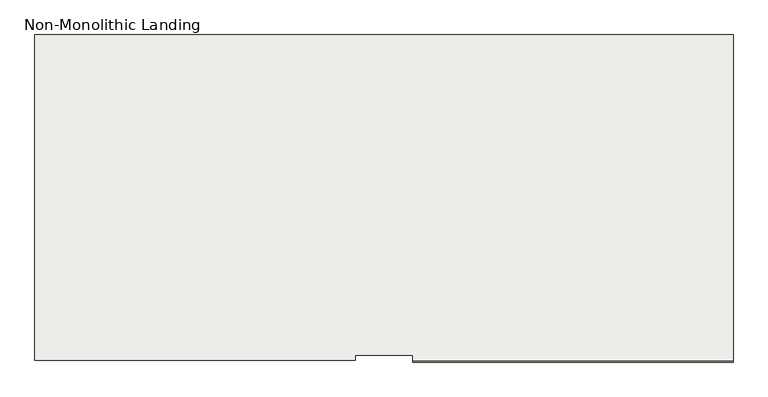
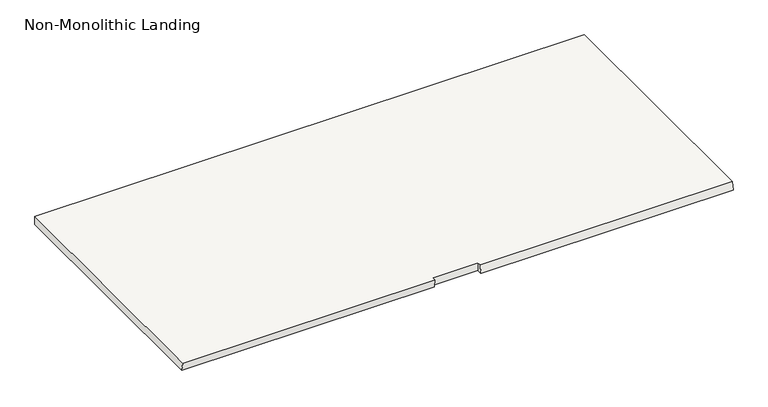
"""IFC4 building model written with IfcOpenShell, lengths in millimetres: slab geometry, Non-Monolithic Landing."""

from ifc_helpers import new_model, si_unit, origin, place, context, project, spatial, faceted_brep, source, transform, mapped, element, save


def non_monolithic_landing_3f935088(model_context):
    return source(origin(), model_context, "Body", "Brep", [
        faceted_brep([(-226.7120949, 7307.4781803, 5617.6470588), (-226.7120949, 7300.3948469, 5567.6470588), (1293.2879051, 7300.3948469, 5567.6470588), (1293.2879051, 7307.4781803, 5617.6470588), (-499.4393676, 7309.7509075, 5617.6470588), (-499.4393676, 7332.4781803, 5617.6470588), (-226.7120949, 7332.4781803, 5617.6470588), (1293.2879051, 7332.4781803, 5617.6470588), (1293.2879051, 8852.4781803, 5617.6470588), (-2019.4393676, 8852.4781803, 5617.6470588), (-2019.4393676, 7309.7509075, 5617.6470588), (-226.7120949, 7332.4781803, 5567.6470588), (-499.4393676, 7332.4781803, 5567.6470588), (-499.4393676, 7316.8342409, 5567.6470588), (-2019.4393676, 7316.8342409, 5567.6470588), (-2019.4393676, 8852.4781803, 5567.6470588), (1293.2879051, 8852.4781803, 5567.6470588), (1293.2879051, 7332.4781803, 5567.6470588)], [[[0, 1, 2, 3]], [[4, 5, 6, 0, 3, 7, 8, 9, 10]], [[11, 12, 13, 14, 15, 16, 17, 2, 1]], [[5, 4, 13, 12]], [[6, 5, 12, 11]], [[0, 6, 11, 1]], [[7, 3, 2, 17]], [[8, 7, 17, 16]], [[9, 8, 16, 15]], [[10, 9, 15, 14]], [[4, 10, 14, 13]]]),
    ])


if __name__ == "__main__":
    model = new_model("IFC4")
    model_context = context("Model", 3, world=origin())
    ifc_project = project(units=[si_unit("LENGTHUNIT", "METRE", prefix="MILLI")], contexts=[model_context])
    site = spatial("IfcSite", under=ifc_project)
    building = spatial("IfcBuilding", under=site)
    placement = place(None, origin())
    non_monolithic_landing_shape = non_monolithic_landing_3f935088(model_context)
    element("IfcSlab", 1, ObjectType="Non-Monolithic Landing", at=placement, inside=building, context=model_context, shape_type="MappedRepresentation", body=[
        mapped(non_monolithic_landing_shape, transform((0.0, 0.0, 0.0), x_axis=(1.0, 0.0, 0.0), y_axis=(0.0, 1.0, 0.0), z_axis=(0.0, 0.0, 1.0))),
    ])
    save(model, "model.ifc")
